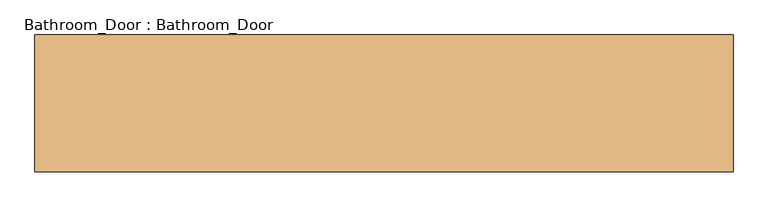
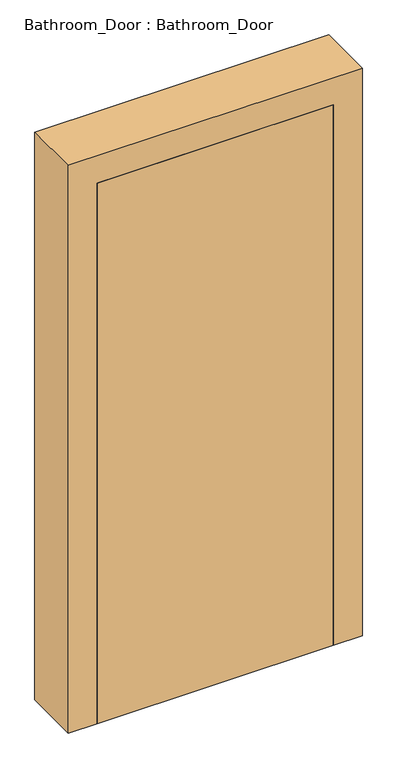
"""IFC4 building model written with IfcOpenShell, lengths in millimetres: door geometry, Bathroom_Door : Bathroom_Door."""

import ifcopenshell
import ifcopenshell.guid

model = None  # the IFC model being written
_history = None  # IfcOwnerHistory: only IFC2X3 demands one
_inside = {}  # id of a spatial element -> (the spatial element, [elements in it])
_under = {}  # id of a project, library or spatial element -> (it, [spatial elements below it])
_declared = {}  # id of a project -> (the project, [libraries it declares])
_typed = {}  # id of a type object -> (the type object, [elements of that type])
_made_of = {}  # id of a material, layer set ... -> (it, [elements and type objects made of it])


def new_model(schema):
    """Start an empty IFC model of exactly this schema.

    Asked for "IFC4X3", IfcOpenShell would pick the latest addendum, in which some entities
    have other attributes; the version numbers below select the first issue.
    IFC2X3 requires an IfcOwnerHistory on every rooted entity: one is made here for all.
    """
    global model, _history
    if schema == "IFC4X3":
        model = ifcopenshell.file(schema_version=(4, 3, 0, 0))
    else:
        model = ifcopenshell.file(schema=schema)
    _inside.clear()
    _under.clear()
    _declared.clear()
    _typed.clear()
    _made_of.clear()
    _history = None
    if model.schema == "IFC2X3":
        org = make("IfcOrganization", Name="unknown")
        user = make(
            "IfcPersonAndOrganization",
            ThePerson=make("IfcPerson", FamilyName="unknown"),
            TheOrganization=org,
        )
        app = make(
            "IfcApplication",
            ApplicationDeveloper=org,
            Version="unknown",
            ApplicationFullName="unknown",
            ApplicationIdentifier="unknown",
        )
        _history = make(
            "IfcOwnerHistory",
            OwningUser=user,
            OwningApplication=app,
            ChangeAction="ADDED",
            CreationDate=0,
        )
    return model


def make(cls, **values):
    """One entity of the class cls with the attributes given. An attribute that is None is left unset."""
    return model.create_entity(
        cls, **{name: value for name, value in values.items() if value is not None}
    )


def rooted(cls, **values):
    """An entity with a GlobalId (a new one), such as an element, a storey or a relation."""
    return make(cls, GlobalId=ifcopenshell.guid.new(), OwnerHistory=_history, **values)


def si_unit(unit_type, name, prefix=None):
    """IfcSIUnit, for example si_unit("LENGTHUNIT", "METRE", prefix="MILLI")."""
    return make("IfcSIUnit", UnitType=unit_type, Prefix=prefix, Name=name)


def assignment(units):
    """IfcUnitAssignment: the units of a project."""
    return None if units is None else make("IfcUnitAssignment", Units=units)


def point(xyz):
    """IfcCartesianPoint."""
    return None if xyz is None else make("IfcCartesianPoint", Coordinates=xyz)


def direction(xyz):
    """IfcDirection."""
    return None if xyz is None else make("IfcDirection", DirectionRatios=xyz)


def frame(location, z_axis=None, x_axis=None):
    """IfcAxis2Placement3D, a coordinate frame: its origin and axes. An axis left out is left unset."""
    return make(
        "IfcAxis2Placement3D",
        Location=point(location),
        Axis=direction(z_axis),
        RefDirection=direction(x_axis),
    )


def origin():
    """The frame at (0, 0, 0) with its axes left unset."""
    return frame((0.0, 0.0, 0.0))


def place(relative_to, where):
    """IfcLocalPlacement: puts the frame where relative to a parent placement (None: the world)."""
    return make(
        "IfcLocalPlacement", PlacementRelTo=relative_to, RelativePlacement=where
    )


def context(
    kind, dimensions, precision=None, world=None, true_north=None, identifier=None
):
    """IfcGeometricRepresentationContext, for example the 3D "Model" context."""
    return make(
        "IfcGeometricRepresentationContext",
        ContextIdentifier=identifier,
        ContextType=kind,
        CoordinateSpaceDimension=dimensions,
        Precision=precision,
        WorldCoordinateSystem=world,
        TrueNorth=true_north,
    )


def project(units=None, contexts=None):
    """IfcProject with its units and contexts."""
    return rooted(
        "IfcProject",
        Name="project",
        RepresentationContexts=contexts,
        UnitsInContext=assignment(units),
    )


def spatial(cls, under=None, at=None, **own):
    """A site, building, storey or space (cls), placed at a placement, below another one or the project."""
    s = rooted(cls, ObjectPlacement=at, **own)
    if under is not None:
        _under.setdefault(under.id(), (under, []))[1].append(s)
    return s


def polyline(points):
    """IfcPolyline through the points."""
    return make("IfcPolyline", Points=[point(p) for p in points])


def outline(outer, holes=None, kind="AREA"):
    """IfcArbitraryClosedProfileDef: a profile drawn as a closed curve; with holes, ...WithVoids."""
    if holes is None:
        return make("IfcArbitraryClosedProfileDef", ProfileType=kind, OuterCurve=outer)
    return make(
        "IfcArbitraryProfileDefWithVoids",
        ProfileType=kind,
        OuterCurve=outer,
        InnerCurves=holes,
    )


def extrude(swept, where, along, depth):
    """IfcExtrudedAreaSolid: the profile swept, set in the frame where, extruded along a direction by depth."""
    return make(
        "IfcExtrudedAreaSolid",
        SweptArea=swept,
        Position=where,
        ExtrudedDirection=direction(along),
        Depth=depth,
    )


def shape(context_of_items, identifier, shape_type, items):
    """IfcShapeRepresentation: the items that make up one representation, for example the "Body"."""
    return make(
        "IfcShapeRepresentation",
        ContextOfItems=context_of_items,
        RepresentationIdentifier=identifier,
        RepresentationType=shape_type,
        Items=items,
    )


def source(mapping_origin, context_of_items, identifier, shape_type, items):
    """IfcRepresentationMap: a shape defined once, which mapped items show again and again."""
    return make(
        "IfcRepresentationMap",
        MappingOrigin=mapping_origin,
        MappedRepresentation=shape(context_of_items, identifier, shape_type, items),
    )


def transform(
    local_origin,
    x_axis=None,
    y_axis=None,
    z_axis=None,
    scale=None,
    scale2=None,
    scale3=None,
    uniform=True,
):
    """IfcCartesianTransformationOperator3D, or its non-uniform kind. x_axis, y_axis, z_axis: its Axis1, 2, 3."""
    if uniform:
        return make(
            "IfcCartesianTransformationOperator3D",
            Axis1=direction(x_axis),
            Axis2=direction(y_axis),
            LocalOrigin=point(local_origin),
            Scale=scale,
            Axis3=direction(z_axis),
        )
    return make(
        "IfcCartesianTransformationOperator3DnonUniform",
        Axis1=direction(x_axis),
        Axis2=direction(y_axis),
        LocalOrigin=point(local_origin),
        Scale=scale,
        Axis3=direction(z_axis),
        Scale2=scale2,
        Scale3=scale3,
    )


def mapped(mapping_source, mapping_target):
    """IfcMappedItem: shows the shape of a source again, moved by a transform."""
    return make(
        "IfcMappedItem", MappingSource=mapping_source, MappingTarget=mapping_target
    )


def made_of(thing, what):
    """Note that an element or type object is made of a material, layer set ...; save() writes the relation."""
    if what is not None:
        _made_of.setdefault(what.id(), (what, []))[1].append(thing)
    return thing


def element(
    cls,
    number,
    at=None,
    inside=None,
    cuts=None,
    type_object=None,
    material=None,
    context=None,
    identifier="Body",
    shape_type=None,
    held_by="IfcProductDefinitionShape",
    body=None,
    shapes=None,
    **own,
):
    """One element of the class cls, such as IfcWall. Its Tag is "e" and its number.

    at: its placement. inside: the storey or other place that contains it. cuts: it is an
    opening in that element (IfcRelVoidsElement). A single representation is given by context,
    identifier, shape_type and body (its items); several are given by shapes. held_by: the class
    of the entity that holds the representations. save() writes the other relations.
    """
    e = rooted(cls, Tag="e%d" % number, ObjectPlacement=at, **own)
    if body is not None:
        shapes = [shape(context, identifier, shape_type, body)]
    if shapes is not None:
        e.Representation = make(held_by, Representations=shapes)
    if inside is not None:
        _inside.setdefault(inside.id(), (inside, []))[1].append(e)
    if cuts is not None:
        rooted(
            "IfcRelVoidsElement", RelatingBuildingElement=cuts, RelatedOpeningElement=e
        )
    if type_object is not None:
        _typed.setdefault(type_object.id(), (type_object, []))[1].append(e)
    return made_of(e, material)


def aggregate(whole, parts):
    """IfcRelAggregates: a whole, such as a stair, and the parts it consists of."""
    return rooted("IfcRelAggregates", RelatingObject=whole, RelatedObjects=parts)


def save(model, path):
    """Write the relations noted so far, then the file.

    IfcRelAggregates (storeys below a building ...), IfcRelContainedInSpatialStructure (elements
    in a storey), IfcRelDefinesByType, IfcRelAssociatesMaterial and IfcRelDeclares: one each for
    every whole, place, type object, material and project.
    """
    for whole, parts in _under.values():
        aggregate(whole, parts)
    for where, things in _inside.values():
        rooted(
            "IfcRelContainedInSpatialStructure",
            RelatedElements=things,
            RelatingStructure=where,
        )
    for kind, things in _typed.values():
        rooted("IfcRelDefinesByType", RelatedObjects=things, RelatingType=kind)
    for what, things in _made_of.values():
        rooted("IfcRelAssociatesMaterial", RelatedObjects=things, RelatingMaterial=what)
    for by, libraries in _declared.values():
        rooted("IfcRelDeclares", RelatingContext=by, RelatedDefinitions=libraries)
    model.write(path)


def bathroom_door_bathroom_door_15b6a89a(model_context):
    return source(origin(), model_context, "Body", "SweptSolid", [
        extrude(outline(polyline([(4275.0, 14755.0), (5095.0, 14755.0), (5095.0, 14655.0), (4275.0, 14655.0), (4275.0, 14755.0)])), frame((0.0, 0.0, 250.0), z_axis=(0.0, 0.0, 1.0), x_axis=(1.0, 0.0, 0.0)), (0.0, 0.0, 1.0), 1980.0),
        extrude(outline(polyline([(250.0, 4175.0), (250.0, 4275.0), (2230.0, 4275.0), (2230.0, 5095.0), (250.0, 5095.0), (250.0, 5195.0), (2330.0, 5195.0), (2330.0, 4175.0), (250.0, 4175.0)])), frame((0.0, 14655.0, 0.0), z_axis=(0.0, 1.0, 0.0), x_axis=(0.0, 0.0, 1.0)), (0.0, 0.0, 1.0), 200.0),
    ])


if __name__ == "__main__":
    model = new_model("IFC4")
    model_context = context("Model", 3, world=origin())
    ifc_project = project(units=[si_unit("LENGTHUNIT", "METRE", prefix="MILLI")], contexts=[model_context])
    site = spatial("IfcSite", under=ifc_project)
    building = spatial("IfcBuilding", under=site)
    placement = place(None, origin())
    bathroom_door_bathroom_door_shape = bathroom_door_bathroom_door_15b6a89a(model_context)
    element("IfcDoor", 1, ObjectType="Bathroom_Door : Bathroom_Door", at=placement, inside=building, context=model_context, shape_type="MappedRepresentation", body=[
        mapped(bathroom_door_bathroom_door_shape, transform((0.0, 0.0, 0.0), x_axis=(1.0, 0.0, 0.0), y_axis=(0.0, 1.0, 0.0), z_axis=(0.0, 0.0, 1.0))),
    ])
    save(model, "model.ifc")

# Revit data of these elements
# Type "Bathroom_Door : Bathroom_Door"
#   Type Mark = "52"
#   NameOverride = "Bathroom_Door"
# Element 1 (IfcDoor, "Bathroom_Door : Bathroom_Door")
#   Materials on its faces: "IfcSurfaceStyle #392"
# Materials
#   "IfcSurfaceStyle #392": class "Unassigned", colour RGB 204 204 204, transparency 0
